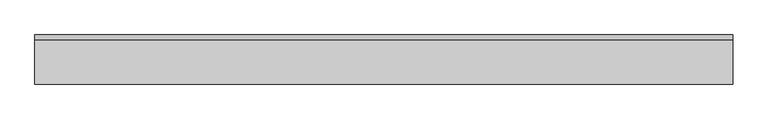
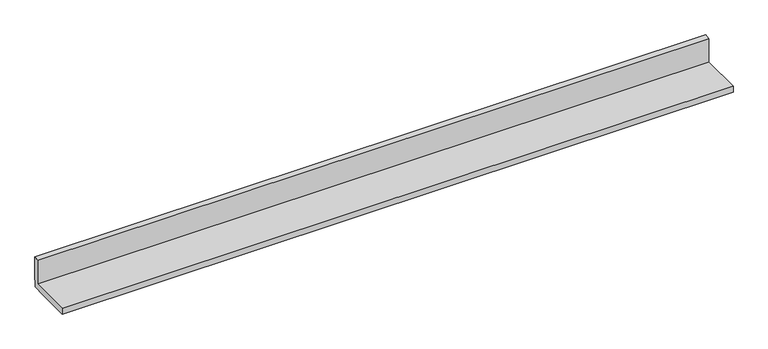
"""IFC4 building model written with IfcOpenShell, lengths in millimetres: proxy geometry, Gypsum017 33610 : Gypsum017 33610."""

from ifc_helpers import new_model, si_unit, frame, origin, place, context, project, spatial, polyline, outline, extrude, source, transform, mapped, element, save


def generic_models_1a790526(model_context):
    return source(origin(), model_context, "Body", "SweptSolid", [
        extrude(outline(polyline([(-4376.7836914, 42583.1921875), (-4376.7836914, 42601.896), (-4250.2279008, 42601.896), (-4250.2279008, 42675.5351562), (-4235.9495263, 42678.9921875), (-4235.9495263, 42605.6253714), (-4237.2648904, 42605.6253714), (-4237.2648904, 42584.4721875), (-4258.4180743, 42584.4721875), (-4258.4180743, 42583.1921875), (-4376.7836914, 42583.1921875)])), frame((12383.0178845, 0.0, 0.0), z_axis=(1.0, 0.0, 0.0), x_axis=(0.0, 1.0, 0.0)), (0.0, 0.0, 1.0), 2000.0),
    ])


if __name__ == "__main__":
    model = new_model("IFC4")
    model_context = context("Model", 3, world=origin())
    ifc_project = project(units=[si_unit("LENGTHUNIT", "METRE", prefix="MILLI")], contexts=[model_context])
    site = spatial("IfcSite", under=ifc_project)
    building = spatial("IfcBuilding", under=site)
    placement = place(None, origin())
    generic_models_shape = generic_models_1a790526(model_context)
    element("IfcBuildingElementProxy", 1, Name="Gypsum017 33610 : Gypsum017 33610", ObjectType="Gypsum017 33610 : Gypsum017 33610", at=placement, inside=building, context=model_context, shape_type="MappedRepresentation", body=[
        mapped(generic_models_shape, transform((0.0, 0.0, 0.0), x_axis=(1.0, 0.0, 0.0), y_axis=(0.0, 1.0, 0.0), z_axis=(0.0, 0.0, 1.0))),
    ])
    save(model, "model.ifc")

# Revit data of these elements
# Type "Gypsum017 33610 : Gypsum017 33610"
#   NameOverride = "Gypsum017"
# Element 1 (IfcBuildingElementProxy, "Gypsum017 33610 : Gypsum017 33610")
#   Materials on its faces: "5/8\"  GYPSUM BOARD"
# Materials
#   "5/8\"  GYPSUM BOARD": class "Unassigned", colour RGB 255 255 255, transparency 0, Cost = 0
